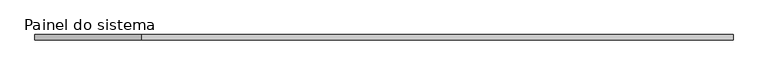
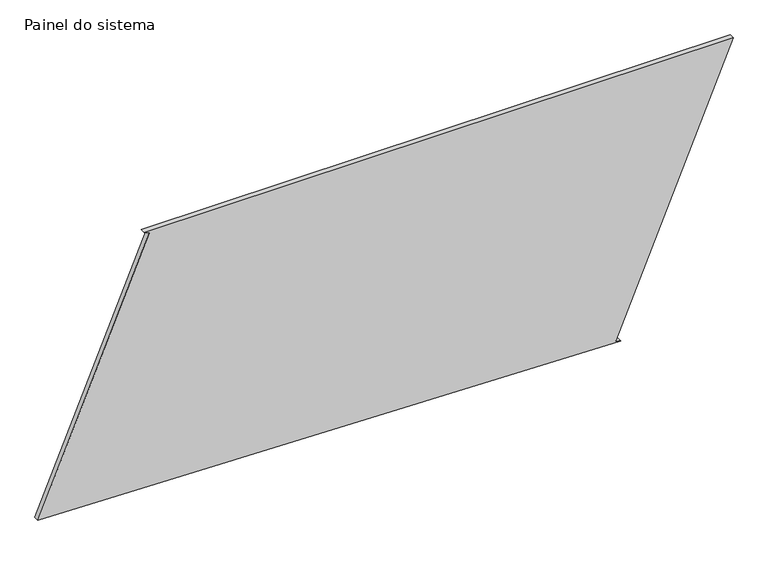
"""IFC4 building model written with IfcOpenShell, lengths in millimetres: plate geometry, Painel do sistema : Envidraçado."""

from ifc_helpers import new_model, si_unit, frame, origin, place, context, project, spatial, polyline, outline, extrude, source, transform, mapped, element, save


def painel_do_sistema_4d27fabb(model_context):
    return source(origin(), model_context, "Body", "SweptSolid", [
        extrude(outline(polyline([(0.0, 1103.6982283), (9.6723918, 1080.6451409), (1320.4437051, 1630.6059109), (1320.4437051, -1132.179066), (1310.7713133, -1109.1259787), (67.8809602, -1630.6059109), (0.0, 1103.6982283)])), frame((0.0, 24.5, 0.0), z_axis=(0.0, 1.0, 0.0), x_axis=(0.0, 0.0, 1.0)), (0.0, 0.0, 1.0), 25.0),
    ])


if __name__ == "__main__":
    model = new_model("IFC4")
    model_context = context("Model", 3, world=origin())
    ifc_project = project(units=[si_unit("LENGTHUNIT", "METRE", prefix="MILLI")], contexts=[model_context])
    site = spatial("IfcSite", under=ifc_project)
    building = spatial("IfcBuilding", under=site)
    placement = place(None, origin())
    painel_do_sistema_shape = painel_do_sistema_4d27fabb(model_context)
    element("IfcPlate", 1, ObjectType="Painel do sistema : Envidraçado", at=placement, inside=building, context=model_context, shape_type="MappedRepresentation", body=[
        mapped(painel_do_sistema_shape, transform((0.0, 0.0, 0.0), x_axis=(1.0, 0.0, 0.0), y_axis=(0.0, 1.0, 0.0), z_axis=(0.0, 0.0, 1.0))),
    ])
    save(model, "model.ifc")

# Revit data of these elements
# Type "Painel do sistema : Envidraçado"
#   Construction Type Id = "GSP4R"
#   Analytic Construction = "Vidraça única Pilkington 1/8 pol"
#   Visual Light Transmittance = 0.9
#   Solar Heat Gain Coefficient = 0.86
#   Heat Transfer Coefficient (U) = 6.7069 W/(m²·K)
# Element 1 (IfcPlate, "Painel do sistema : Envidraçado")
#   Materials on its faces: "Vidro"
# Materials
#   "Vidro": class "Vidro", colour RGB 0 128 192, transparency 0.9, Description = "Vidro de sílica", Cost = 0
